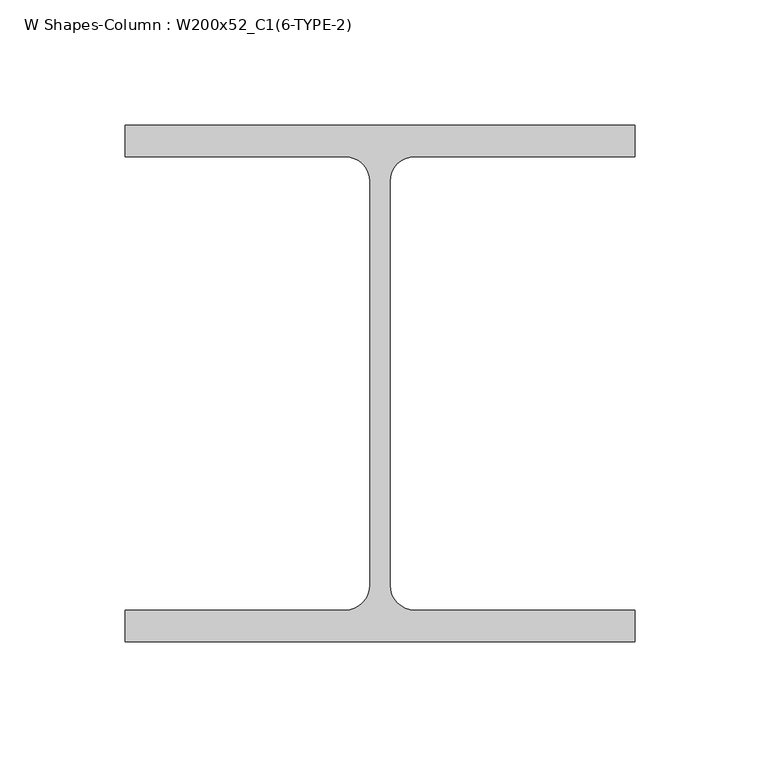
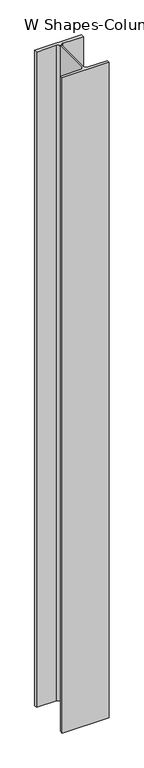
"""IFC4 building model written with IfcOpenShell, lengths in millimetres: column geometry, W Shapes-Column : W200x52_C1(6-TYPE-2)."""

from ifc_helpers import new_model, si_unit, point, frame, frame_2d, origin, place, context, project, spatial, polyline, circle_curve, trimmed, segment, composite_curve, outline, extrude, source, transform, mapped, element, save


def w_shapes_column_w200x52_c1_6_type_2_b3dfbed1(model_context):
    return source(origin(), model_context, "Body", "SweptSolid", [
        extrude(outline(composite_curve([segment(polyline([(101.854, 103.124), (101.854, 90.551), (13.9446, 90.551)]), True, "CONTINUOUS"), segment(trimmed(circle_curve(frame_2d((13.9446, 80.5434)), 10.0076), [point((13.9446, 90.551))], [point((3.937, 80.5434))], True, "CARTESIAN"), True, "CONTINUOUS"), segment(polyline([(3.937, 80.5434), (3.937, -80.5434)]), True, "CONTINUOUS"), segment(trimmed(circle_curve(frame_2d((13.9446, -80.5434)), 10.0076), [point((3.937, -80.5434))], [point((13.9446, -90.551))], True, "CARTESIAN"), True, "CONTINUOUS"), segment(polyline([(13.9446, -90.551), (101.854, -90.551), (101.854, -103.124), (-101.854, -103.124), (-101.854, -90.551), (-13.9446, -90.551)]), True, "CONTINUOUS"), segment(trimmed(circle_curve(frame_2d((-13.9446, -80.5434)), 10.0076), [point((-13.9446, -90.551))], [point((-3.937, -80.5434))], True, "CARTESIAN"), True, "CONTINUOUS"), segment(polyline([(-3.937, -80.5434), (-3.937, 80.5434)]), True, "CONTINUOUS"), segment(trimmed(circle_curve(frame_2d((-13.9446, 80.5434)), 10.0076), [point((-3.937, 80.5434))], [point((-13.9446, 90.551))], True, "CARTESIAN"), True, "CONTINUOUS"), segment(polyline([(-13.9446, 90.551), (-101.854, 90.551), (-101.854, 103.124), (101.854, 103.124)]), True, "CONTINUOUS")], self_intersect=False)), frame((0.0, 0.0, 6240.0), z_axis=(0.0, 0.0, 1.0), x_axis=(1.0, 0.0, 0.0)), (0.0, 0.0, 1.0), 3000.0),
    ])


if __name__ == "__main__":
    model = new_model("IFC4")
    model_context = context("Model", 3, world=origin())
    ifc_project = project(units=[si_unit("LENGTHUNIT", "METRE", prefix="MILLI")], contexts=[model_context])
    site = spatial("IfcSite", under=ifc_project)
    building = spatial("IfcBuilding", under=site)
    placement = place(None, origin())
    w_shapes_column_w200x52_c1_6_type_2_shape = w_shapes_column_w200x52_c1_6_type_2_b3dfbed1(model_context)
    element("IfcColumn", 1, ObjectType="W Shapes-Column : W200x52_C1(6-TYPE-2)", at=placement, inside=building, context=model_context, shape_type="MappedRepresentation", body=[
        mapped(w_shapes_column_w200x52_c1_6_type_2_shape, transform((0.0, 0.0, 0.0), x_axis=(1.0, 0.0, 0.0), y_axis=(0.0, 1.0, 0.0), z_axis=(0.0, 0.0, 1.0))),
    ])
    save(model, "model.ifc")

# Revit data of these elements
# Type "W Shapes-Column : W200x52_C1(6-TYPE-2)"
#   Section Name Key = "W8X35"
#   Assembly Code = "B10"
#   Width = 20.3708 cm
#   Web Thickness = 0.7874 cm
#   Web Fillet = 1.0008 cm
#   Warping Constant = 166223.7 cm⁶
#   Torsional Moment of Inertia = 32.0082 cm⁴
#   Section Area = 66.4515 cm²
#   Plastic Modulus weak axis = 263.832 cm³
#   Plastic Modulus strong axis = 568.631 cm³
#   Perimeter = 1.1936 m²/m
#   Nominal Weight = 52.0857 kgf/m
#   Moment of Inertia weak axis = 1773.15 cm⁴
#   Moment of Inertia strong axis = 5286.14 cm⁴
#   Height = 20.6248 cm
#   Flange Thickness = 1.2573 cm
#   Elastic Modulus weak axis = 173.703 cm³
#   Elastic Modulus strong axis = 511.276 cm³
#   Clear Web Height = 14.605 cm
#   Centroid Vertical = 10.3124 cm
#   Centroid Horizontal = 10.1854 cm
#   Bolt Spacing = 13.97 cm
#   Structural Material [instance default] = Steel ASTM A992
#   Principal Axes Angle = 0
# Element 1 (IfcColumn, "W Shapes-Column : W200x52_C1(6-TYPE-2)")
#   Structural Material = none
# Materials
#   "Steel ASTM A992": class "Metal", colour RGB 199 199 199, transparency 0, Description = "Structural steel 50ksi", Cost = 0
